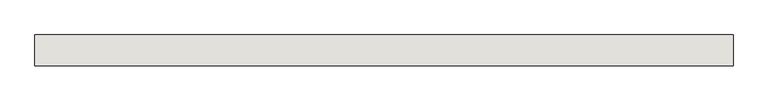
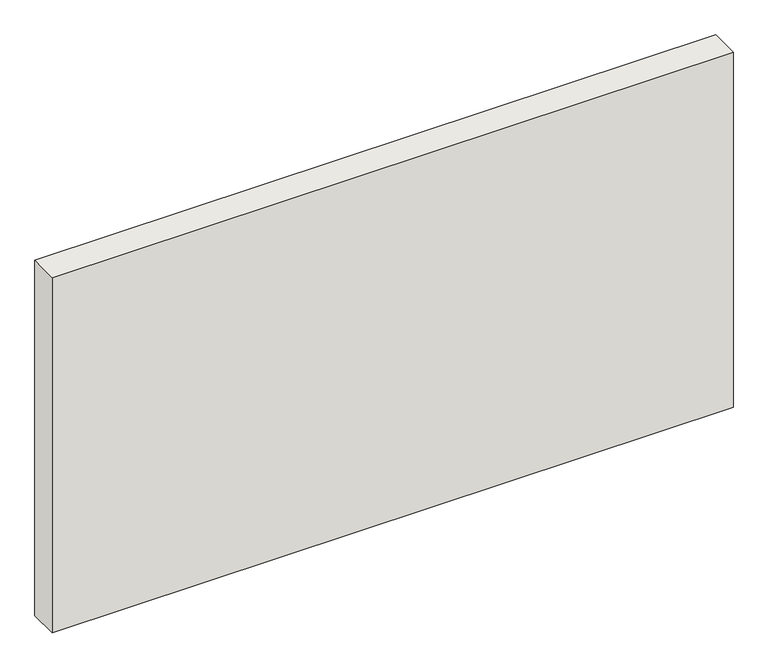
"""IFC4 building model written with IfcOpenShell, lengths in millimetres: wall geometry, Holzwand."""

from ifc_helpers import new_model, si_unit, origin, origin_with_axes, place, context, project, spatial, polyline, outline, extrude, source, transform, mapped, element, save


def wall_17cb042b(model_context):
    return source(origin(), model_context, "Body", "SweptSolid", [
        extrude(outline(polyline([(0.0, 200.0), (4550.0, 200.0), (4550.0, 0.0), (0.0, 0.0), (0.0, 200.0)])), origin_with_axes(), (0.0, 0.0, 1.0), 2510.0),
    ])


if __name__ == "__main__":
    model = new_model("IFC4")
    model_context = context("Model", 3, world=origin())
    ifc_project = project(units=[si_unit("LENGTHUNIT", "METRE", prefix="MILLI")], contexts=[model_context])
    site = spatial("IfcSite", under=ifc_project)
    building = spatial("IfcBuilding", under=site)
    placement = place(None, origin())
    wall_shape = wall_17cb042b(model_context)
    element("IfcWall", 1, ObjectType="Holzwand", at=placement, inside=building, context=model_context, shape_type="MappedRepresentation", body=[
        mapped(wall_shape, transform((0.0, 0.0, 0.0), x_axis=(1.0, 0.0, 0.0), y_axis=(0.0, 1.0, 0.0), z_axis=(0.0, 0.0, 1.0))),
    ])
    save(model, "model.ifc")

# Revit data of these elements
# Element 1 (IfcWall, "Holzwand")
#   Materials on its faces: "holzschalung"
# Materials
#   "holzschalung": class "Unassigned", colour RGB 128 128 128, transparency 0
